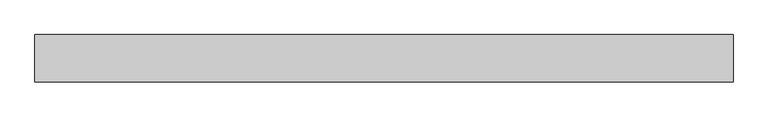
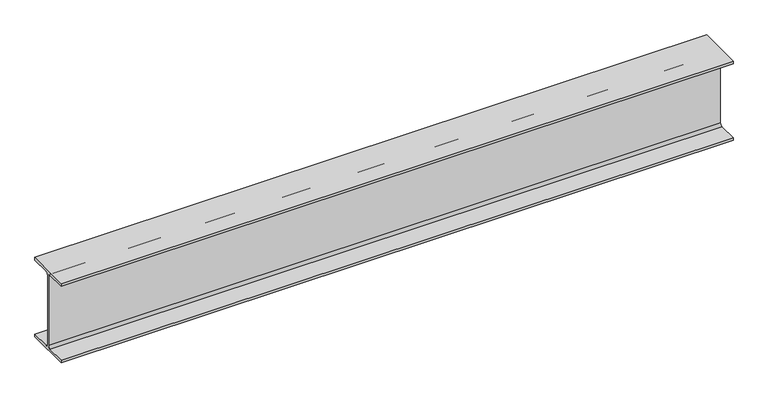
"""IFC4 building model written with IfcOpenShell, lengths in millimetres: beam geometry, Old_Steel Beam_H-KSD3502 : H_SB_ASB_H-200×200x8x12."""

from ifc_helpers import new_model, si_unit, point, frame, frame_2d, origin, place, context, project, spatial, polyline, circle_curve, trimmed, segment, composite_curve, outline, extrude, source, transform, mapped, element, save


def beam_3d9c44e8(model_context):
    return source(origin(), model_context, "Body", "SweptSolid", [
        extrude(outline(composite_curve([segment(polyline([(82.5, -141.5), (82.5, -151.7), (-82.5, -151.7), (-82.5, -141.5), (-11.9, -141.5)]), True, "CONTINUOUS"), segment(trimmed(circle_curve(frame_2d((-11.9, -132.6)), 8.9), [point((-11.9, -141.5))], [point((-3.0, -132.6))], True, "CARTESIAN"), True, "CONTINUOUS"), segment(polyline([(-3.0, -132.6), (-3.0, 132.6)]), True, "CONTINUOUS"), segment(trimmed(circle_curve(frame_2d((-11.9, 132.6)), 8.9), [point((-3.0, 132.6))], [point((-11.9, 141.5))], True, "CARTESIAN"), True, "CONTINUOUS"), segment(polyline([(-11.9, 141.5), (-82.5, 141.5), (-82.5, 151.7), (82.5, 151.7), (82.5, 141.5), (11.9, 141.5)]), True, "CONTINUOUS"), segment(trimmed(circle_curve(frame_2d((11.9, 132.6)), 8.9), [point((11.9, 141.5))], [point((3.0, 132.6))], True, "CARTESIAN"), True, "CONTINUOUS"), segment(polyline([(3.0, 132.6), (3.0, -132.6)]), True, "CONTINUOUS"), segment(trimmed(circle_curve(frame_2d((11.9, -132.6)), 8.9), [point((3.0, -132.6))], [point((11.9, -141.5))], True, "CARTESIAN"), True, "CONTINUOUS"), segment(polyline([(11.9, -141.5), (82.5, -141.5)]), True, "CONTINUOUS")], self_intersect=False)), frame((-1238.7267651, 0.0, 0.0), z_axis=(1.0, 0.0, 0.0), x_axis=(0.0, 1.0, 0.0)), (0.0, 0.0, 1.0), 2428.9452569),
    ])


if __name__ == "__main__":
    model = new_model("IFC4")
    model_context = context("Model", 3, world=origin())
    ifc_project = project(units=[si_unit("LENGTHUNIT", "METRE", prefix="MILLI")], contexts=[model_context])
    site = spatial("IfcSite", under=ifc_project)
    building = spatial("IfcBuilding", under=site)
    placement = place(None, origin())
    beam_shape = beam_3d9c44e8(model_context)
    element("IfcBeam", 1, ObjectType="Old_Steel Beam_H-KSD3502 : H_SB_ASB_H-200×200x8x12", at=placement, inside=building, context=model_context, shape_type="MappedRepresentation", body=[
        mapped(beam_shape, transform((0.0, 0.0, 0.0), x_axis=(1.0, 0.0, 0.0), y_axis=(0.0, 1.0, 0.0), z_axis=(0.0, 0.0, 1.0))),
    ])
    save(model, "model.ifc")

# Revit data of these elements
# Type "Old_Steel Beam_H-KSD3502 : H_SB_ASB_H-200×200x8x12"
#   Width = 20.0 cm
#   Web Thickness = 0.8 cm
#   Web Fillet = 1.3 cm
#   Warping Constant = 141376.0 cm⁶
#   Torsional Moment of Inertia = 26.2485 cm⁴
#   Torsional Modulus = 1.0 cm³
#   Section Area = 63.53 cm²
#   Plastic Modulus weak axis = 244.0 cm³
#   Plastic Modulus strong axis = 525.0 cm³
#   Perimeter = 1.16 m²/m
#   Nominal Weight = 49.90 kgf/m
#   Moment of Inertia weak axis = 1600.00 cm⁴
#   Moment of Inertia strong axis = 4720.00 cm⁴
#   Height = 20.0 cm
#   Flange Thickness = 1.2 cm
#   Elastic Modulus weak axis = 160.0 cm³
#   Elastic Modulus strong axis = 472.0 cm³
#   Centroid Vertical = 10.0 cm
#   Centroid Horizontal = 10.0 cm
#   Length [instance default] = 1.5240 m
#   Structural Material [instance default] = Steel, 45-345
#   Assembly Code = ""
# Element 1 (IfcBeam, "Old_Steel Beam_H-KSD3502 : H_SB_ASB_H-200×200x8x12")
#   Structural Material = none
# Materials
#   "Steel, 45-345": class "Metal", colour RGB 189 187 185, transparency 0, Description = "Steel 345 MPa", Cost = 0
